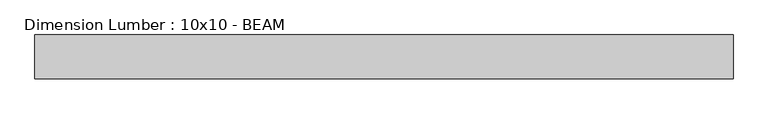
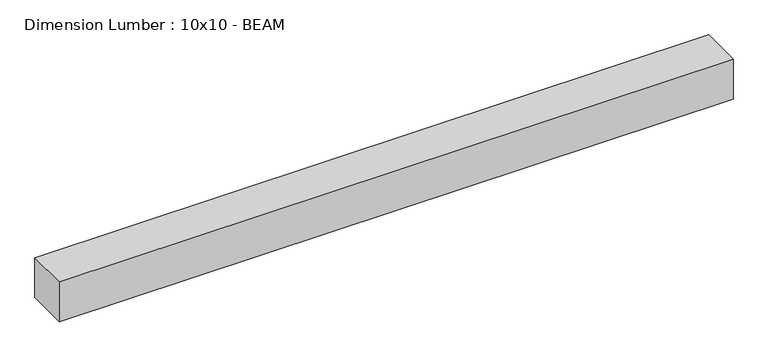
"""IFC4 building model written with IfcOpenShell, lengths in millimetres: beam geometry, Dimension Lumber : 10x10 - BEAM."""

from ifc_helpers import new_model, si_unit, frame, origin, place, context, project, spatial, polyline, outline, extrude, source, transform, mapped, element, save


def dimension_lumber_10x10_beam_470fd3cf(model_context):
    return source(origin(), model_context, "Body", "SweptSolid", [
        extrude(outline(polyline([(1876.3363558, 117.475), (1876.3363558, -117.475), (-1876.3363558, -117.475), (-1876.3363558, 117.475), (1876.3363558, 117.475)])), frame((0.0, 0.0, -117.475), z_axis=(0.0, 0.0, 1.0), x_axis=(1.0, 0.0, 0.0)), (0.0, 0.0, 1.0), 234.95),
    ])


if __name__ == "__main__":
    model = new_model("IFC4")
    model_context = context("Model", 3, world=origin())
    ifc_project = project(units=[si_unit("LENGTHUNIT", "METRE", prefix="MILLI")], contexts=[model_context])
    site = spatial("IfcSite", under=ifc_project)
    building = spatial("IfcBuilding", under=site)
    placement = place(None, origin())
    dimension_lumber_10x10_beam_shape = dimension_lumber_10x10_beam_470fd3cf(model_context)
    element("IfcBeam", 1, ObjectType="Dimension Lumber : 10x10 - BEAM", at=placement, inside=building, context=model_context, shape_type="MappedRepresentation", body=[
        mapped(dimension_lumber_10x10_beam_shape, transform((0.0, 0.0, 0.0), x_axis=(1.0, 0.0, 0.0), y_axis=(0.0, 1.0, 0.0), z_axis=(0.0, 0.0, 1.0))),
    ])
    save(model, "model.ifc")

# Revit data of these elements
# Type "Dimension Lumber : 10x10 - BEAM"
#   Assembly Code = "B10"
#   A = 0.0755556 SF
#   Length [instance default] = 5' - 0"
#   b = 0' - 9 1/4"
#   d = 0' - 9 1/4"
#   Structural Material = (4) CHARRED SISTERED 2X10s AT BEAM
# Element 1 (IfcBeam, "Dimension Lumber : 10x10 - BEAM")
#   Materials on its faces: "(4) CHARRED SISTERED 2X10s AT BEAM"
# Materials
#   "(4) CHARRED SISTERED 2X10s AT BEAM": class "Wood", colour RGB 144 144 144, transparency 0, Description = "Pinus Echinata", Cost = 0
